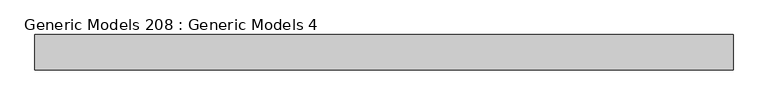
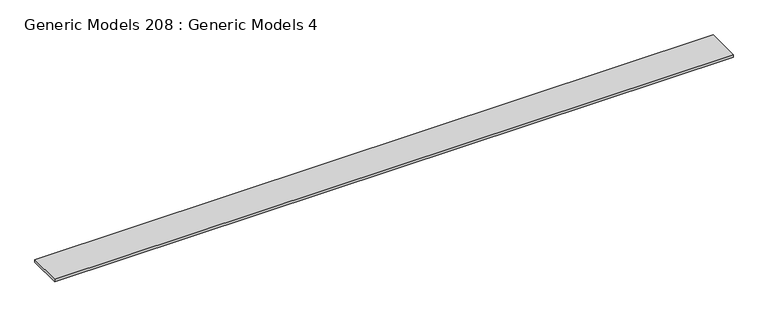
"""IFC4 building model written with IfcOpenShell, lengths in millimetres: proxy geometry, Generic Models 208 : Generic Models 4."""

from ifc_helpers import new_model, si_unit, frame, origin, place, context, project, spatial, polyline, outline, extrude, source, transform, mapped, element, save


def generic_models_208_generic_models_4_d9dc6814(model_context):
    return source(origin(), model_context, "Body", "SweptSolid", [
        extrude(outline(polyline([(-19489.9914237, 6242.3269221), (-19489.9914237, 6877.3269221), (-6942.3914237, 6877.3269221), (-6942.3914237, 6242.3269221), (-19489.9914237, 6242.3269221)])), frame((0.0, 0.0, 122958.228424), z_axis=(0.0, 0.0, 1.0), x_axis=(1.0, 0.0, 0.0)), (0.0, 0.0, 1.0), 50.8),
    ])


if __name__ == "__main__":
    model = new_model("IFC4")
    model_context = context("Model", 3, world=origin())
    ifc_project = project(units=[si_unit("LENGTHUNIT", "METRE", prefix="MILLI")], contexts=[model_context])
    site = spatial("IfcSite", under=ifc_project)
    building = spatial("IfcBuilding", under=site)
    placement = place(None, origin())
    generic_models_208_generic_models_4_shape = generic_models_208_generic_models_4_d9dc6814(model_context)
    element("IfcBuildingElementProxy", 1, Name="Generic Models 208 : Generic Models 4", ObjectType="Generic Models 208 : Generic Models 4", at=placement, inside=building, context=model_context, shape_type="MappedRepresentation", body=[
        mapped(generic_models_208_generic_models_4_shape, transform((0.0, 0.0, 0.0), x_axis=(1.0, 0.0, 0.0), y_axis=(0.0, 1.0, 0.0), z_axis=(0.0, 0.0, 1.0))),
    ])
    save(model, "model.ifc")

# Revit data of these elements
# Element 1 (IfcBuildingElementProxy, "Generic Models 208 : Generic Models 4")
#   Materials on its faces: "_2\" SAND"
# Materials
#   "_2\" SAND": class "Generic", colour RGB 245 226 173, transparency 0, Cost = 0
